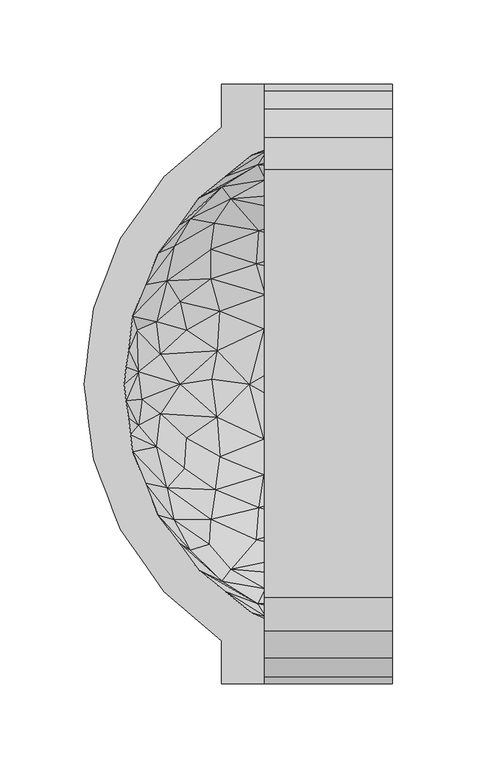
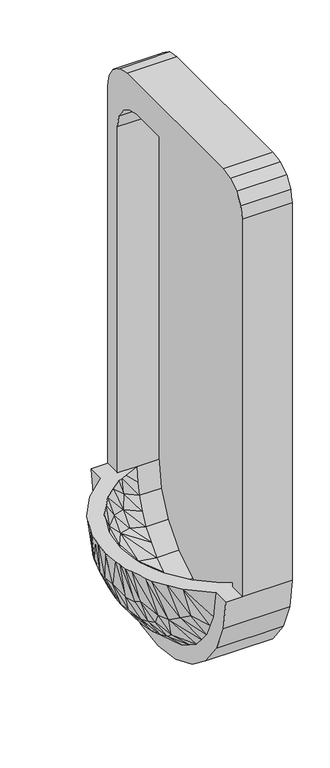
"""IFC4 building model written with IfcOpenShell, lengths in millimetres: proxy geometry, Urinal-Wall-3D:Urinal-Wall-3D:2446:Urinal-Wall-3D:2446 : Urinal-Wall-3D:Urinal-Wall-3D:2446:300505 : Urinal-Wall-3D:Urinal-Wall-3D:2446:Urinal-Wall-3D:2446 : Urinal-Wall-3D:Urinal-Wall-3D:2446:300505."""

from ifc_helpers import new_model, si_unit, origin, place, context, project, spatial, triangles, source, transform, mapped, element, save


def generic_models_7ac7ee6e(model_context):
    return source(origin(), model_context, "Body", "Tessellation", [
        triangles([(647621.4931641, -573335.0135742, 609.6), (647612.1914062, -573307.9268555, 609.6), (647599.2433594, -573326.2699219, 609.6), (647595.1505859, -573336.7250977, 609.6), (647645.0824219, -573272.3941406, 609.6), (647625.0650391, -573289.5837891, 609.6), (647645.5289063, -573302.4574219, 609.6), (647633.4738281, -573318.7168945, 609.6), (647613.9029297, -573353.765918, 609.6), (647587.1138672, -573357.6726563, 609.6), (647606.3871094, -573372.5554688, 609.6), (647591.1322266, -573347.2174805, 609.6), (647581.6816406, -573379.2899414, 609.6), (647583.0210938, -573368.127832, 609.6), (647603.8570313, -573392.6100586, 609.6), (647580.2677734, -573390.4148438, 609.6), (647602.5175781, -573402.655957, 609.6), (647578.9283203, -573401.5397461, 609.6), (647684.521875, -573234.8894531, 609.6), (647659.1466797, -573234.8894531, 609.6), (647684.521875, -573260.3018555, 609.6), (647659.1466797, -573260.3018555, 609.6), (647677.0060547, -573277.0078125, 609.6), (647661.2302734, -573289.7326172, 609.6), (647713.8410156, -573260.3018555, 609.6), (647690.8470703, -573270.7198242, 609.6), (647683.9265625, -573273.8824219, 609.6), (647605.1220703, -573382.6013672, 609.6), (647601.2525391, -573412.7018555, 609.6), (647577.5144531, -573412.7018555, 609.6), (647578.9283203, -573423.8267578, 609.6), (647580.2677734, -573434.9516602, 609.6), (647602.5175781, -573422.7105469, 609.6), (647603.8570313, -573432.7564453, 609.6), (647605.1220703, -573442.8023438, 609.6), (647581.6816406, -573446.1137695, 609.6), (647606.3871094, -573452.8482422, 609.6), (647583.0210938, -573457.2386719, 609.6), (647587.1138672, -573467.6938477, 609.6), (647613.9029297, -573471.6005859, 609.6), (647591.1322266, -573478.1862305, 609.6), (647595.1505859, -573488.6414063, 609.6), (647621.4931641, -573490.3901367, 609.6), (647599.2433594, -573499.1337891, 609.6), (647612.1914062, -573517.4768555, 609.6), (647633.4738281, -573506.6496094, 609.6), (647645.5289063, -573522.9462891, 609.6), (647625.0650391, -573535.8199219, 609.6), (647661.2302734, -573535.6710938, 609.6), (647645.0824219, -573553.0095703, 609.6), (647690.8470703, -573554.6466797, 609.6), (647677.0060547, -573548.3958984, 609.6), (647684.521875, -573565.1018555, 609.6), (647659.1466797, -573565.1018555, 609.6), (647659.1466797, -573590.4770508, 609.6), (647702.3068359, -573559.8556641, 609.6), (647713.8410156, -573565.1018555, 609.6), (647684.521875, -573590.4770508, 609.6), (647685.8613281, -573274.2544922, 583.9469873), (647659.2955078, -573529.6807617, 571.4722764), (647713.8410156, -573331.144043, 482.6979349), (647713.8410156, -573312.8753906, 494.4237817), (647681.3220703, -573321.7306641, 505.4282335), (647664.8765625, -573522.5370117, 545.0935813), (647685.1171875, -573533.9967773, 538.9458097), (647713.8410156, -573526.7041992, 510.8150414), (647609.8101563, -573405.4836914, 558.6713862), (647664.8765625, -573302.8294922, 545.0936176), (647713.8410156, -573298.6995117, 510.8150414), (647685.1171875, -573291.3697266, 538.9458097), (647713.8410156, -573494.259668, 482.6979349), (647679.8337891, -573505.1241211, 507.9383274), (647713.8410156, -573512.4911133, 494.4237817), (647684.4474609, -573379.9224609, 473.4506433), (647685.3404297, -573359.793457, 479.4091822), (647658.1792969, -573369.5416992, 495.410422), (647656.6166016, -573392.9821289, 490.4112722), (647675.5921875, -573412.7018555, 474.7844645), (647713.8410156, -573266.4782227, 566.663958), (647713.8410156, -573263.6504883, 586.2369638), (647680.6523438, -573282.402832, 564.4870923), (647659.2955078, -573295.7229492, 571.4722764), (647638.3851562, -573380.7782227, 512.4167241), (647622.9070313, -573395.0657227, 531.3763953), (647638.3851562, -573444.6999023, 512.4541128), (647622.9070313, -573430.1891602, 531.3513605), (647620.6746094, -573449.7972656, 543.0548249), (647679.8337891, -573341.2271484, 492.2453536), (647658.1792969, -573455.8620117, 495.410422), (647684.4474609, -573466.3916016, 480.2694131), (647684.3730469, -573445.3324219, 473.4754601), (647630.7949219, -573493.2550781, 564.2788201), (647626.7021484, -573474.1306641, 548.7818009), (647640.8408203, -573314.5869141, 571.7064554), (647637.1945313, -573462.6708984, 522.0602489), (647685.8613281, -573551.1120117, 583.9469873), (647680.6523438, -573543.0008789, 564.4870923), (647713.8410156, -573284.4864258, 527.2063374), (647713.8410156, -573275.4823242, 546.9351477), (647652.0773438, -573507.8402344, 542.0659318), (647655.0539063, -573317.1169922, 538.0613434), (647652.7470703, -573332.6323242, 523.79539), (647713.8410156, -573549.9213867, 546.9351477), (647681.3220703, -573485.9625, 492.3042526), (647713.8410156, -573475.9910156, 470.9720881), (647609.8845703, -573437.0724609, 563.910783), (647608.9916016, -573380.7410156, 572.3650998), (647631.1669922, -573331.0324219, 565.2611003), (647626.7021484, -573351.2730469, 548.7818009), (647713.8410156, -573558.9254883, 566.663958), (647713.8410156, -573563.4275391, 597.9184819), (647713.8410156, -573561.7160156, 586.2369638), (647713.8410156, -573349.3754883, 470.9720881), (647640.5431641, -573511.1888672, 573.9630401), (647655.4259766, -573475.5073242, 507.6571309), (647713.8410156, -573391.0101562, 458.7512135), (647713.8410156, -573412.7018555, 458.7512135), (647713.8410156, -573434.3935547, 458.7512135), (647713.8410156, -573540.8800781, 527.2063374), (647620.6746094, -573375.6064453, 543.0548249), (647713.8410156, -573370.1742187, 464.8616326), (647611.89375, -573421.7431641, 553.1137676), (647634.4412109, -573412.7018555, 512.2263288), (647656.4677734, -573432.347168, 490.5842631), (647634.5900391, -573363.7001953, 525.2664122), (647652.7470703, -573492.7713867, 523.79539), (647652.7470703, -573350.23125, 510.2499232), (647653.3423828, -573409.799707, 491.7342293), (647713.8410156, -573455.1922852, 464.8616326), (647747.9970703, -573266.4782227, 566.663958), (647747.9970703, -573260.3018555, 609.6), (647747.9970703, -573284.4864258, 527.2063374), (647747.9970703, -573349.3754883, 470.9720881), (647747.9970703, -573312.8753906, 494.4237817), (647747.9970703, -573391.0101562, 458.7512135), (647747.9970703, -573434.3935547, 458.7512135), (647747.9970703, -573475.9910156, 470.9720881), (647747.9970703, -573512.4911133, 494.4237817), (647747.9970703, -573565.1018555, 609.6), (647747.9970703, -573558.9254883, 566.663958), (647747.9970703, -573540.8800781, 527.2063374), (647760.721875, -573549.4004883, 1268.066494), (647760.721875, -573559.1487305, 1266.1330364), (647760.721875, -573567.3714844, 1260.6271225), (647760.721875, -573588.5422852, 1228.9201916), (647760.721875, -573539.6894531, 1269.9999516), (647760.721875, -573581.1008789, 1246.8807232), (647760.721875, -573575.5942383, 1255.1210632), (647760.721875, -573234.8894531, 1219.2), (647760.721875, -573285.6770508, 1269.9999516), (647760.721875, -573257.9950195, 1260.6271225), (647760.721875, -573275.9660156, 1268.066494), (647760.721875, -573244.265625, 1246.8807232), (647760.721875, -573266.2549805, 1266.1330364), (647760.721875, -573236.8242188, 1228.9201916), (647760.721875, -573249.7722656, 1255.1210632), (647760.721875, -573238.7589844, 1238.6403831), (647760.721875, -573586.6075195, 1238.6403831), (647760.721875, -573590.4770508, 1219.2), (647760.721875, -573584.4495117, 563.5819877), (647760.721875, -573234.8894531, 609.6), (647760.721875, -573590.4770508, 609.6), (647760.721875, -573258.7019531, 520.7000121), (647760.721875, -573566.6645508, 520.7000121), (647760.721875, -573538.4244141, 483.876424), (647760.721875, -573501.5894531, 455.6206996), (647760.721875, -573286.9792969, 483.876424), (647760.721875, -573240.9541992, 563.5819877), (647760.721875, -573458.7269531, 437.8583754), (647760.721875, -573323.7770508, 455.6206996), (647760.721875, -573366.6767578, 437.8583754), (647760.721875, -573412.7018555, 431.7999879), (647659.1466797, -573240.9541992, 563.5819877), (647659.1466797, -573286.9792969, 483.876424), (647659.1466797, -573258.7019531, 520.7000121), (647659.1466797, -573323.7770508, 455.6206996), (647659.1466797, -573366.6767578, 437.8583754), (647659.1466797, -573412.7018555, 431.7999879), (647659.1466797, -573458.7269531, 437.8583754), (647659.1466797, -573501.5894531, 455.6206996), (647659.1466797, -573566.6645508, 520.7000121), (647659.1466797, -573584.4495117, 563.5819877), (647659.1466797, -573538.4244141, 483.876424), (647659.1466797, -573412.7018555, 458.7512135), (647659.1466797, -573434.3935547, 458.7512135), (647659.1466797, -573391.0101562, 458.7512135), (647659.1466797, -573494.259668, 482.6979349), (647659.1466797, -573475.9910156, 470.9720881), (647659.1466797, -573512.4911133, 494.4237817), (647659.1466797, -573455.1922852, 464.8616326), (647659.1466797, -573370.1742187, 464.8616326), (647659.1466797, -573349.3754883, 470.9720881), (647659.1466797, -573331.144043, 482.6979349), (647659.1466797, -573312.8753906, 494.4237817), (647659.1466797, -573298.6995117, 510.8150414), (647659.1466797, -573284.4864258, 527.2063374), (647659.1466797, -573549.9213867, 546.9351477), (647659.1466797, -573540.8800781, 527.2063374), (647659.1466797, -573526.7041992, 510.8150414), (647659.1466797, -573562.0136719, 588.2859303), (647659.1466797, -573558.9254883, 566.663958), (647659.1466797, -573275.4823242, 546.9351477), (647659.1466797, -573266.4782227, 566.663958), (647659.1466797, -573263.352832, 588.2859303), (647636.5248047, -573339.9993164, 496.2975772), (647629.2322266, -573357.7842773, 494.5229762), (647612.3402344, -573340.4458008, 530.1853706), (647635.7806641, -573286.5328125, 564.7131323), (647606.6847656, -573354.8821289, 529.1428834), (647627.5207031, -573325.3397461, 519.1144621), (647604.6011719, -573332.1486328, 557.7764917), (647618.7398438, -573315.1450195, 547.3545261), (647626.8509766, -573299.2204102, 557.2311399), (647630.94375, -573445.2580078, 484.5077808), (647630.94375, -573380.1084961, 484.5077808), (647594.9273438, -573349.5987305, 563.8420009), (647606.9080078, -573389.7451172, 512.8612101), (647585.4767578, -573397.5958008, 558.5052627), (647589.4951172, -573379.2527344, 553.8611421), (647626.8509766, -573526.1833008, 557.2311399), (647635.7806641, -573538.8708984, 564.7131323), (647630.94375, -573465.9451172, 491.8173274), (647607.9498047, -573455.1178711, 517.92133), (647612.3402344, -573484.9579102, 530.1853706), (647633.1761719, -573480.9767578, 497.2734624), (647631.6134766, -573494.6689453, 508.7941981), (647592.9925781, -573464.2708008, 557.1740939), (647589.1230469, -573447.899707, 555.9720234), (647625.7347656, -573425.3522461, 486.402905), (647600.8804688, -573434.6912109, 522.8274985), (647602.0710938, -573412.7018555, 518.0100964), (647627.7439453, -573402.5071289, 484.0731417), (647583.7652344, -573422.3756836, 563.1875713), (647607.9498047, -573370.2858398, 517.92133), (647590.4625, -573362.2491211, 564.5393057), (647609.4380859, -573496.715332, 549.5402212), (647594.8529297, -573475.9910156, 564.3948741), (647618.7398438, -573510.2586914, 547.3544898), (647609.8845703, -573469.7774414, 522.8140182), (647684.521875, -573565.1018555, 1168.3999758), (647684.521875, -573563.390332, 1176.8655928), (647684.521875, -573590.4770508, 1219.2), (647684.521875, -573561.2323242, 1187.8402863), (647684.521875, -573550.219043, 1204.321039), (647684.521875, -573555.7256836, 1196.080699), (647684.521875, -573567.3714844, 1260.6271225), (647684.521875, -573533.7363281, 1215.3330849), (647684.521875, -573541.959082, 1209.8270256), (647684.521875, -573524.025293, 1217.2665424), (647684.521875, -573539.6894531, 1269.9999516), (647684.521875, -573581.1008789, 1246.8807232), (647684.521875, -573262.2366211, 1178.1201674), (647684.521875, -573264.1713867, 1187.8402863), (647684.521875, -573234.8894531, 1219.2), (647684.521875, -573260.3018555, 1168.3999758), (647684.521875, -573291.6673828, 1215.3330849), (647684.521875, -573302.643457, 1217.5160912), (647684.521875, -573285.6770508, 1269.9999516), (647684.521875, -573244.265625, 1246.8807232), (647684.521875, -573275.184668, 1204.321039), (647684.521875, -573283.4074219, 1209.8270256), (647684.521875, -573269.6780273, 1196.080699), (647684.521875, -573257.9950195, 1260.6271225), (647684.521875, -573588.5422852, 1228.9201916), (647684.521875, -573586.6075195, 1238.6403831), (647684.521875, -573559.1487305, 1266.1330364), (647684.521875, -573546.7587891, 1268.5966942), (647684.521875, -573514.2770508, 1219.2), (647684.521875, -573575.5942383, 1255.1210632), (647684.521875, -573311.0894531, 1219.2), (647684.521875, -573238.7589844, 1238.6403831), (647684.521875, -573236.3033203, 1226.2546566), (647684.521875, -573275.9660156, 1268.066494), (647684.521875, -573249.7722656, 1255.1210632), (647684.521875, -573266.2549805, 1266.1330364), (647747.9970703, -573260.3018555, 1168.3999758), (647747.9970703, -573264.1713867, 1187.8402863), (647747.9970703, -573261.9761719, 1176.8655928), (647747.9970703, -573275.184668, 1204.321039), (647747.9970703, -573269.6780273, 1196.080699), (647747.9970703, -573291.6673828, 1215.3330849), (647747.9970703, -573301.378418, 1217.2665424), (647747.9970703, -573311.0894531, 1219.2), (647747.9970703, -573283.4074219, 1209.8270256), (647747.9970703, -573514.2770508, 1219.2), (647747.9970703, -573533.7363281, 1215.3330849), (647747.9970703, -573522.7602539, 1217.5160912), (647747.9970703, -573550.219043, 1204.321039), (647747.9970703, -573541.959082, 1209.8270256), (647747.9970703, -573561.2323242, 1187.8402863), (647747.9970703, -573563.1670898, 1178.1201674), (647747.9970703, -573565.1018555, 1168.3999758), (647747.9970703, -573555.7256836, 1196.080699)], [[1, 2, 3], [1, 3, 4], [5, 6, 7], [2, 8, 6], [1, 8, 2], [4, 9, 1], [9, 10, 11], [9, 12, 10], [13, 11, 14], [10, 14, 11], [15, 13, 16], [17, 16, 18], [12, 9, 4], [19, 20, 21], [21, 20, 22], [23, 22, 24], [21, 22, 23], [25, 21, 26], [27, 26, 21], [21, 23, 27], [7, 6, 8], [15, 28, 13], [11, 13, 28], [24, 22, 5], [17, 15, 16], [17, 18, 29], [24, 5, 7], [18, 30, 29], [31, 32, 33], [31, 33, 29], [33, 32, 34], [36, 35, 34], [35, 36, 37], [36, 34, 32], [31, 29, 30], [38, 39, 37], [37, 39, 40], [40, 41, 42], [39, 41, 40], [40, 42, 43], [43, 42, 44], [38, 37, 36], [43, 45, 46], [45, 43, 44], [47, 46, 48], [49, 47, 50], [51, 52, 53], [49, 54, 52], [45, 48, 46], [49, 50, 54], [54, 55, 53], [54, 53, 52], [57, 56, 53], [58, 53, 55], [56, 51, 53], [50, 47, 48], [59, 23, 24], [46, 47, 60], [61, 62, 63], [64, 65, 66], [29, 67, 17], [15, 17, 67], [68, 69, 70], [71, 72, 73], [74, 75, 76], [74, 77, 78], [79, 80, 27], [80, 26, 27], [25, 26, 80], [70, 81, 82], [7, 81, 24], [77, 83, 84], [85, 86, 87], [61, 63, 88], [89, 90, 91], [40, 92, 93], [94, 8, 1], [89, 85, 95], [96, 49, 52], [97, 60, 47], [7, 82, 81], [81, 98, 99], [72, 100, 64], [63, 101, 102], [96, 103, 97], [71, 104, 72], [71, 105, 104], [86, 106, 87], [15, 107, 28], [11, 28, 107], [108, 109, 102], [52, 110, 96], [56, 57, 111], [51, 56, 112], [52, 112, 110], [52, 51, 112], [112, 56, 111], [113, 61, 88], [64, 100, 114], [90, 89, 115], [79, 27, 59], [116, 78, 117], [118, 117, 78], [47, 49, 97], [8, 94, 82], [60, 65, 64], [8, 82, 7], [70, 82, 68], [119, 65, 97], [81, 70, 98], [62, 69, 68], [69, 98, 70], [114, 60, 64], [60, 97, 65], [64, 66, 73], [65, 119, 66], [109, 11, 120], [59, 99, 79], [97, 103, 119], [121, 75, 74], [33, 106, 122], [84, 83, 120], [87, 106, 35], [123, 122, 86], [85, 89, 124], [120, 83, 125], [92, 43, 114], [102, 101, 108], [109, 9, 11], [93, 126, 115], [93, 37, 40], [24, 81, 59], [99, 59, 81], [103, 96, 110], [97, 49, 96], [59, 27, 23], [74, 116, 121], [91, 124, 89], [102, 88, 63], [62, 68, 63], [68, 101, 63], [102, 127, 88], [127, 76, 75], [68, 94, 101], [108, 1, 9], [108, 101, 94], [109, 108, 9], [127, 102, 109], [125, 109, 120], [77, 74, 76], [88, 75, 113], [78, 116, 74], [83, 77, 76], [128, 78, 77], [113, 75, 121], [75, 88, 127], [94, 68, 82], [108, 94, 1], [76, 127, 125], [107, 84, 120], [67, 123, 84], [77, 84, 123], [76, 125, 83], [127, 109, 125], [104, 115, 126], [104, 105, 90], [104, 126, 72], [100, 72, 126], [64, 73, 72], [92, 100, 126], [100, 92, 114], [93, 92, 126], [40, 43, 92], [91, 129, 118], [129, 91, 90], [118, 78, 91], [124, 91, 78], [128, 124, 78], [86, 85, 124], [90, 105, 129], [90, 115, 104], [115, 89, 95], [43, 46, 114], [60, 114, 46], [86, 124, 123], [95, 87, 93], [67, 122, 123], [33, 34, 106], [35, 106, 34], [87, 95, 85], [115, 95, 93], [86, 122, 106], [35, 37, 87], [67, 29, 33], [37, 93, 87], [33, 122, 67], [107, 67, 84], [77, 123, 128], [11, 107, 120], [15, 67, 107], [124, 128, 123], [79, 130, 80], [80, 131, 25], [131, 80, 130], [132, 130, 99], [79, 99, 130], [99, 98, 132], [113, 133, 61], [61, 134, 62], [134, 61, 133], [62, 134, 69], [69, 132, 98], [132, 69, 134], [116, 135, 121], [121, 133, 113], [133, 121, 135], [135, 116, 117], [117, 118, 136], [117, 136, 135], [137, 105, 71], [71, 73, 138], [71, 138, 137], [136, 118, 129], [129, 105, 137], [129, 137, 136], [111, 57, 139], [112, 139, 140], [139, 112, 111], [112, 140, 110], [103, 140, 141], [140, 103, 110], [103, 141, 119], [66, 141, 138], [141, 66, 119], [66, 138, 73], [142, 143, 144], [145, 146, 142], [142, 147, 145], [144, 148, 147], [142, 144, 147], [149, 150, 146], [153, 151, 152], [151, 154, 152], [155, 152, 150], [153, 156, 151], [155, 157, 153], [152, 155, 153], [149, 155, 150], [145, 147, 158], [149, 146, 159], [160, 161, 162], [149, 159, 162], [163, 164, 165], [165, 166, 167], [160, 164, 168], [166, 169, 170], [164, 163, 168], [160, 168, 161], [161, 149, 162], [169, 171, 170], [167, 166, 170], [165, 167, 163], [171, 169, 172], [159, 146, 145], [19, 168, 173], [168, 19, 161], [19, 173, 20], [174, 175, 167], [163, 167, 175], [176, 174, 170], [167, 170, 174], [173, 168, 163], [163, 175, 173], [177, 176, 171], [170, 171, 176], [178, 177, 172], [171, 172, 177], [169, 179, 172], [178, 172, 179], [169, 166, 180], [180, 179, 169], [181, 164, 182], [160, 182, 164], [164, 181, 165], [183, 165, 181], [165, 183, 166], [180, 166, 183], [160, 162, 58], [58, 55, 182], [58, 182, 160], [184, 178, 185], [184, 186, 178], [178, 179, 185], [178, 186, 177], [180, 187, 188], [189, 187, 180], [190, 185, 179], [179, 188, 190], [179, 180, 188], [177, 191, 192], [191, 177, 186], [176, 192, 193], [192, 176, 177], [194, 174, 176], [174, 195, 175], [195, 174, 194], [195, 196, 175], [194, 176, 193], [181, 197, 198], [197, 181, 182], [199, 181, 198], [181, 199, 183], [182, 55, 200], [182, 200, 201], [200, 55, 54], [182, 201, 197], [199, 189, 183], [202, 173, 175], [203, 204, 173], [204, 20, 173], [20, 204, 22], [202, 203, 173], [202, 175, 196], [189, 180, 183], [6, 5, 204], [6, 204, 203], [22, 204, 5], [205, 206, 207], [208, 202, 196], [206, 209, 207], [210, 211, 212], [3, 2, 213], [214, 185, 190], [6, 202, 208], [191, 215, 206], [213, 212, 3], [6, 203, 202], [205, 207, 210], [211, 216, 10], [217, 218, 219], [220, 221, 45], [197, 201, 48], [214, 222, 223], [201, 200, 48], [200, 50, 48], [54, 50, 200], [2, 208, 213], [224, 225, 226], [227, 36, 228], [229, 230, 231], [198, 197, 221], [205, 193, 192], [221, 48, 45], [232, 229, 231], [221, 220, 198], [233, 231, 230], [219, 218, 16], [215, 217, 234], [234, 235, 209], [217, 215, 232], [224, 236, 237], [227, 237, 38], [189, 238, 226], [208, 196, 213], [2, 6, 208], [212, 195, 194], [195, 212, 213], [193, 210, 194], [212, 211, 4], [213, 196, 195], [48, 221, 197], [220, 45, 44], [238, 220, 44], [238, 199, 220], [236, 42, 41], [236, 41, 39], [187, 226, 225], [189, 199, 238], [199, 198, 220], [226, 236, 224], [206, 205, 192], [210, 207, 211], [215, 234, 206], [206, 234, 209], [194, 210, 212], [193, 205, 210], [206, 192, 191], [232, 215, 186], [191, 186, 215], [229, 184, 185], [184, 229, 232], [232, 231, 217], [217, 231, 218], [233, 218, 231], [16, 218, 18], [30, 18, 218], [229, 185, 214], [214, 230, 229], [223, 228, 230], [30, 233, 31], [32, 31, 233], [233, 230, 228], [218, 233, 30], [232, 186, 184], [227, 228, 223], [32, 233, 228], [223, 222, 239], [228, 36, 32], [227, 38, 36], [190, 188, 222], [188, 225, 222], [223, 239, 227], [222, 214, 190], [214, 223, 230], [234, 219, 235], [216, 207, 209], [219, 16, 13], [10, 12, 211], [12, 4, 211], [216, 14, 10], [216, 211, 207], [238, 44, 42], [239, 237, 227], [187, 225, 188], [236, 39, 237], [237, 39, 38], [239, 225, 224], [189, 226, 187], [236, 226, 238], [42, 236, 238], [216, 235, 14], [217, 219, 234], [13, 14, 235], [209, 235, 216], [219, 13, 235], [225, 239, 222], [237, 239, 224], [4, 3, 212], [53, 58, 240], [242, 241, 240], [242, 243, 241], [58, 242, 240], [242, 244, 245], [246, 247, 248], [249, 247, 250], [248, 244, 251], [245, 243, 242], [252, 253, 254], [19, 21, 255], [19, 255, 254], [255, 252, 254], [256, 257, 258], [259, 260, 261], [253, 262, 254], [261, 256, 263], [254, 262, 260], [251, 244, 264], [246, 248, 251], [251, 264, 265], [266, 247, 246], [264, 244, 242], [250, 247, 267], [268, 249, 250], [266, 267, 247], [251, 269, 246], [270, 268, 250], [259, 271, 260], [261, 263, 259], [272, 254, 260], [260, 271, 272], [258, 257, 270], [256, 273, 263], [263, 274, 259], [273, 275, 263], [256, 258, 273], [258, 270, 250], [276, 255, 25], [21, 25, 255], [25, 131, 276], [277, 253, 252], [277, 252, 278], [278, 255, 276], [255, 278, 252], [279, 260, 262], [279, 262, 280], [262, 277, 280], [277, 262, 253], [256, 281, 282], [256, 282, 257], [257, 283, 270], [283, 257, 282], [260, 279, 284], [260, 284, 261], [284, 256, 261], [256, 284, 281], [285, 268, 270], [270, 283, 285], [286, 247, 249], [286, 249, 287], [287, 268, 285], [268, 287, 249], [288, 244, 248], [288, 248, 289], [248, 286, 289], [286, 248, 247], [243, 290, 291], [243, 291, 241], [241, 292, 240], [292, 241, 291], [244, 288, 293], [244, 293, 245], [293, 243, 245], [243, 293, 290], [57, 240, 292], [240, 57, 53], [57, 292, 139], [159, 242, 162], [58, 162, 242], [148, 269, 251], [148, 251, 147], [251, 158, 147], [158, 251, 265], [242, 159, 145], [242, 145, 264], [145, 265, 264], [265, 145, 158], [146, 250, 267], [146, 267, 142], [142, 266, 143], [266, 142, 267], [246, 269, 148], [266, 246, 143], [148, 144, 246], [144, 143, 246], [150, 258, 250], [250, 146, 150], [156, 274, 263], [156, 263, 151], [263, 154, 151], [154, 263, 275], [258, 150, 152], [258, 152, 273], [152, 275, 273], [275, 152, 154], [149, 254, 272], [149, 272, 155], [155, 271, 157], [271, 155, 272], [259, 274, 156], [271, 259, 157], [156, 153, 259], [153, 157, 259], [161, 19, 149], [254, 149, 19], [292, 285, 276], [283, 282, 278], [282, 284, 280], [284, 279, 280], [284, 282, 281], [285, 283, 276], [293, 288, 289], [291, 290, 293], [291, 293, 289], [287, 291, 289], [292, 291, 287], [292, 287, 285], [287, 289, 286], [278, 282, 280], [283, 278, 276], [139, 292, 276], [140, 131, 130], [130, 132, 141], [276, 131, 139], [132, 134, 138], [130, 141, 140], [132, 138, 141], [139, 131, 140], [133, 135, 136], [133, 136, 137], [134, 137, 138], [134, 133, 137], [278, 280, 277]]),
    ])


if __name__ == "__main__":
    model = new_model("IFC4")
    model_context = context("Model", 3, world=origin())
    ifc_project = project(units=[si_unit("LENGTHUNIT", "METRE", prefix="MILLI")], contexts=[model_context])
    site = spatial("IfcSite", under=ifc_project)
    building = spatial("IfcBuilding", under=site)
    placement = place(None, origin())
    generic_models_shape = generic_models_7ac7ee6e(model_context)
    element("IfcBuildingElementProxy", 1, Name="Urinal-Wall-3D:Urinal-Wall-3D:2446:Urinal-Wall-3D:2446 : Urinal-Wall-3D:Urinal-Wall-3D:2446:300505 : Urinal-Wall-3D:Urinal-Wall-3D:2446:Urinal-Wall-3D:2446 : Urinal-Wall-3D:Urinal-Wall-3D:2446:300505", ObjectType="Urinal-Wall-3D:Urinal-Wall-3D:2446:Urinal-Wall-3D:2446 : Urinal-Wall-3D:Urinal-Wall-3D:2446:300505 : Urinal-Wall-3D:Urinal-Wall-3D:2446:Urinal-Wall-3D:2446 : Urinal-Wall-3D:Urinal-Wall-3D:2446:300505", at=placement, inside=building, context=model_context, shape_type="MappedRepresentation", body=[
        mapped(generic_models_shape, transform((0.0, 0.0, 0.0), x_axis=(1.0, 0.0, 0.0), y_axis=(0.0, 1.0, 0.0), z_axis=(0.0, 0.0, 1.0))),
    ])
    save(model, "model.ifc")

# Revit data of these elements
# Type "Urinal-Wall-3D:Urinal-Wall-3D:2446:Urinal-Wall-3D:2446 : Urinal-Wall-3D:Urinal-Wall-3D:2446:300505 : Urinal-Wall-3D:Urinal-Wall-3D:2446:Urinal-Wall-3D:2446 : Urinal-Wall-3D:Urinal-Wall-3D:2446:300505"
#   NameOverride = "Urinal-Wall-3D:Urinal-Wall-3D:2446:Urinal-Wall-3D:2446 : Urinal-Wall-3D:Urinal-Wall-3D:2446:300505"
#   ObjectTypeOverride = "Urinal-Wall-3D:2446 : Urinal-Wall-3D:Urinal-Wall-3D:2446"
#   Tag = "300505"
#   Reference = "Urinal-Wall-3D"
